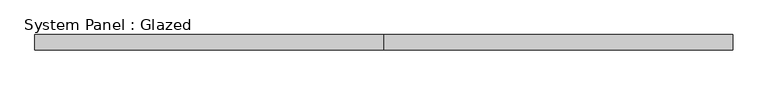
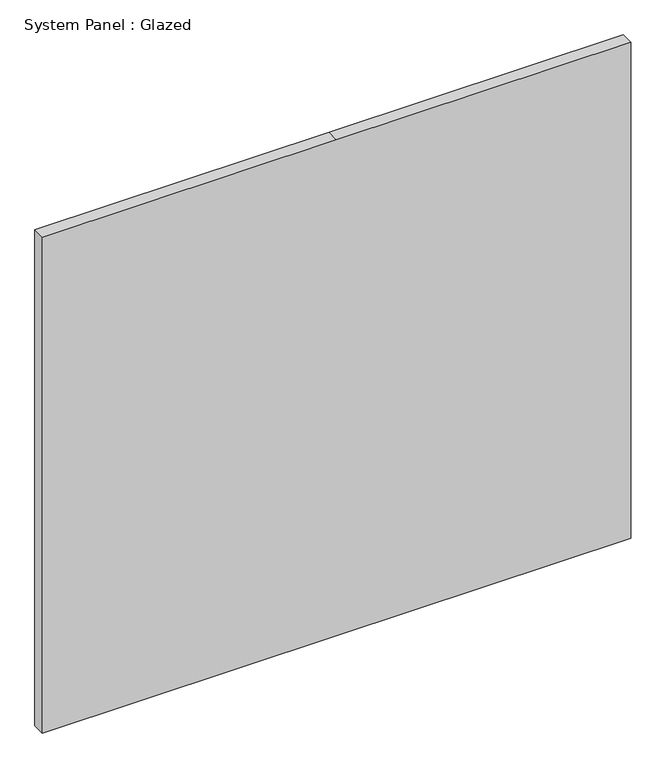
"""IFC4 building model written with IfcOpenShell, lengths in millimetres: plate geometry, System Panel : Glazed."""

from ifc_helpers import new_model, si_unit, frame, origin, place, context, project, spatial, polyline, outline, extrude, source, transform, mapped, element, save


def system_panel_glazed_e8de8d64(model_context):
    return source(origin(), model_context, "Body", "SweptSolid", [
        extrude(outline(polyline([(0.0, -1150.0), (0.0, 0.0), (0.0, 1150.0), (2050.0, 1150.0), (2050.0, 0.0), (2050.0, -1150.0), (0.0, -1150.0)])), frame((0.0, -25.0, 0.0), z_axis=(0.0, 1.0, 0.0), x_axis=(0.0, 0.0, 1.0)), (0.0, 0.0, 1.0), 50.0),
    ])


if __name__ == "__main__":
    model = new_model("IFC4")
    model_context = context("Model", 3, world=origin())
    ifc_project = project(units=[si_unit("LENGTHUNIT", "METRE", prefix="MILLI")], contexts=[model_context])
    site = spatial("IfcSite", under=ifc_project)
    building = spatial("IfcBuilding", under=site)
    placement = place(None, origin())
    system_panel_glazed_shape = system_panel_glazed_e8de8d64(model_context)
    element("IfcPlate", 1, ObjectType="System Panel : Glazed", at=placement, inside=building, context=model_context, shape_type="MappedRepresentation", body=[
        mapped(system_panel_glazed_shape, transform((0.0, 0.0, 0.0), x_axis=(1.0, 0.0, 0.0), y_axis=(0.0, 1.0, 0.0), z_axis=(0.0, 0.0, 1.0))),
    ])
    save(model, "model.ifc")

# Revit data of these elements
# Type "System Panel : Glazed"
#   Type Mark = "CW-GLASS"
# Element 1 (IfcPlate, "System Panel : Glazed")
#   Materials on its faces: "Glass_Clear"
# Materials
#   "Glass_Clear": class "Glass", colour RGB 128 128 255, transparency 0.8, Comments = "Rendering appearance not upgraded ", Cost = 0
